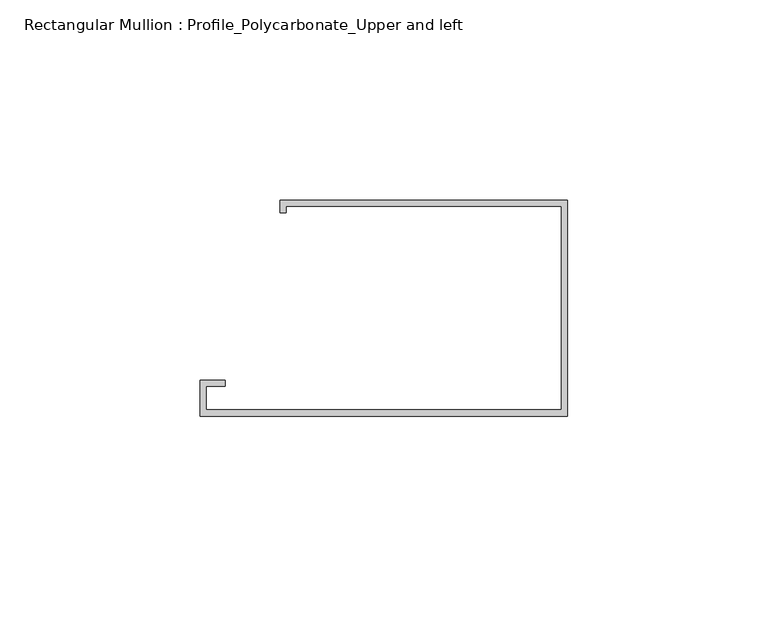
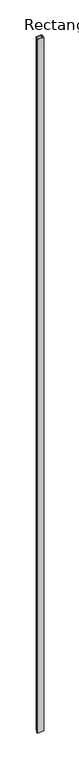
"""IFC4 building model written with IfcOpenShell, lengths in millimetres: member geometry, Rectangular Mullion : Profile_Polycarbonate_Upper and left."""

import ifcopenshell
import ifcopenshell.guid

model = None  # the IFC model being written
_history = None  # IfcOwnerHistory: only IFC2X3 demands one
_inside = {}  # id of a spatial element -> (the spatial element, [elements in it])
_under = {}  # id of a project, library or spatial element -> (it, [spatial elements below it])
_declared = {}  # id of a project -> (the project, [libraries it declares])
_typed = {}  # id of a type object -> (the type object, [elements of that type])
_made_of = {}  # id of a material, layer set ... -> (it, [elements and type objects made of it])


def new_model(schema):
    """Start an empty IFC model of exactly this schema.

    Asked for "IFC4X3", IfcOpenShell would pick the latest addendum, in which some entities
    have other attributes; the version numbers below select the first issue.
    IFC2X3 requires an IfcOwnerHistory on every rooted entity: one is made here for all.
    """
    global model, _history
    if schema == "IFC4X3":
        model = ifcopenshell.file(schema_version=(4, 3, 0, 0))
    else:
        model = ifcopenshell.file(schema=schema)
    _inside.clear()
    _under.clear()
    _declared.clear()
    _typed.clear()
    _made_of.clear()
    _history = None
    if model.schema == "IFC2X3":
        org = make("IfcOrganization", Name="unknown")
        user = make(
            "IfcPersonAndOrganization",
            ThePerson=make("IfcPerson", FamilyName="unknown"),
            TheOrganization=org,
        )
        app = make(
            "IfcApplication",
            ApplicationDeveloper=org,
            Version="unknown",
            ApplicationFullName="unknown",
            ApplicationIdentifier="unknown",
        )
        _history = make(
            "IfcOwnerHistory",
            OwningUser=user,
            OwningApplication=app,
            ChangeAction="ADDED",
            CreationDate=0,
        )
    return model


def make(cls, **values):
    """One entity of the class cls with the attributes given. An attribute that is None is left unset."""
    return model.create_entity(
        cls, **{name: value for name, value in values.items() if value is not None}
    )


def rooted(cls, **values):
    """An entity with a GlobalId (a new one), such as an element, a storey or a relation."""
    return make(cls, GlobalId=ifcopenshell.guid.new(), OwnerHistory=_history, **values)


def si_unit(unit_type, name, prefix=None):
    """IfcSIUnit, for example si_unit("LENGTHUNIT", "METRE", prefix="MILLI")."""
    return make("IfcSIUnit", UnitType=unit_type, Prefix=prefix, Name=name)


def assignment(units):
    """IfcUnitAssignment: the units of a project."""
    return None if units is None else make("IfcUnitAssignment", Units=units)


def point(xyz):
    """IfcCartesianPoint."""
    return None if xyz is None else make("IfcCartesianPoint", Coordinates=xyz)


def direction(xyz):
    """IfcDirection."""
    return None if xyz is None else make("IfcDirection", DirectionRatios=xyz)


def frame(location, z_axis=None, x_axis=None):
    """IfcAxis2Placement3D, a coordinate frame: its origin and axes. An axis left out is left unset."""
    return make(
        "IfcAxis2Placement3D",
        Location=point(location),
        Axis=direction(z_axis),
        RefDirection=direction(x_axis),
    )


def origin():
    """The frame at (0, 0, 0) with its axes left unset."""
    return frame((0.0, 0.0, 0.0))


def place(relative_to, where):
    """IfcLocalPlacement: puts the frame where relative to a parent placement (None: the world)."""
    return make(
        "IfcLocalPlacement", PlacementRelTo=relative_to, RelativePlacement=where
    )


def context(
    kind, dimensions, precision=None, world=None, true_north=None, identifier=None
):
    """IfcGeometricRepresentationContext, for example the 3D "Model" context."""
    return make(
        "IfcGeometricRepresentationContext",
        ContextIdentifier=identifier,
        ContextType=kind,
        CoordinateSpaceDimension=dimensions,
        Precision=precision,
        WorldCoordinateSystem=world,
        TrueNorth=true_north,
    )


def project(units=None, contexts=None):
    """IfcProject with its units and contexts."""
    return rooted(
        "IfcProject",
        Name="project",
        RepresentationContexts=contexts,
        UnitsInContext=assignment(units),
    )


def spatial(cls, under=None, at=None, **own):
    """A site, building, storey or space (cls), placed at a placement, below another one or the project."""
    s = rooted(cls, ObjectPlacement=at, **own)
    if under is not None:
        _under.setdefault(under.id(), (under, []))[1].append(s)
    return s


def polyline(points):
    """IfcPolyline through the points."""
    return make("IfcPolyline", Points=[point(p) for p in points])


def outline(outer, holes=None, kind="AREA"):
    """IfcArbitraryClosedProfileDef: a profile drawn as a closed curve; with holes, ...WithVoids."""
    if holes is None:
        return make("IfcArbitraryClosedProfileDef", ProfileType=kind, OuterCurve=outer)
    return make(
        "IfcArbitraryProfileDefWithVoids",
        ProfileType=kind,
        OuterCurve=outer,
        InnerCurves=holes,
    )


def extrude(swept, where, along, depth):
    """IfcExtrudedAreaSolid: the profile swept, set in the frame where, extruded along a direction by depth."""
    return make(
        "IfcExtrudedAreaSolid",
        SweptArea=swept,
        Position=where,
        ExtrudedDirection=direction(along),
        Depth=depth,
    )


def shape(context_of_items, identifier, shape_type, items):
    """IfcShapeRepresentation: the items that make up one representation, for example the "Body"."""
    return make(
        "IfcShapeRepresentation",
        ContextOfItems=context_of_items,
        RepresentationIdentifier=identifier,
        RepresentationType=shape_type,
        Items=items,
    )


def source(mapping_origin, context_of_items, identifier, shape_type, items):
    """IfcRepresentationMap: a shape defined once, which mapped items show again and again."""
    return make(
        "IfcRepresentationMap",
        MappingOrigin=mapping_origin,
        MappedRepresentation=shape(context_of_items, identifier, shape_type, items),
    )


def transform(
    local_origin,
    x_axis=None,
    y_axis=None,
    z_axis=None,
    scale=None,
    scale2=None,
    scale3=None,
    uniform=True,
):
    """IfcCartesianTransformationOperator3D, or its non-uniform kind. x_axis, y_axis, z_axis: its Axis1, 2, 3."""
    if uniform:
        return make(
            "IfcCartesianTransformationOperator3D",
            Axis1=direction(x_axis),
            Axis2=direction(y_axis),
            LocalOrigin=point(local_origin),
            Scale=scale,
            Axis3=direction(z_axis),
        )
    return make(
        "IfcCartesianTransformationOperator3DnonUniform",
        Axis1=direction(x_axis),
        Axis2=direction(y_axis),
        LocalOrigin=point(local_origin),
        Scale=scale,
        Axis3=direction(z_axis),
        Scale2=scale2,
        Scale3=scale3,
    )


def mapped(mapping_source, mapping_target):
    """IfcMappedItem: shows the shape of a source again, moved by a transform."""
    return make(
        "IfcMappedItem", MappingSource=mapping_source, MappingTarget=mapping_target
    )


def made_of(thing, what):
    """Note that an element or type object is made of a material, layer set ...; save() writes the relation."""
    if what is not None:
        _made_of.setdefault(what.id(), (what, []))[1].append(thing)
    return thing


def element(
    cls,
    number,
    at=None,
    inside=None,
    cuts=None,
    type_object=None,
    material=None,
    context=None,
    identifier="Body",
    shape_type=None,
    held_by="IfcProductDefinitionShape",
    body=None,
    shapes=None,
    **own,
):
    """One element of the class cls, such as IfcWall. Its Tag is "e" and its number.

    at: its placement. inside: the storey or other place that contains it. cuts: it is an
    opening in that element (IfcRelVoidsElement). A single representation is given by context,
    identifier, shape_type and body (its items); several are given by shapes. held_by: the class
    of the entity that holds the representations. save() writes the other relations.
    """
    e = rooted(cls, Tag="e%d" % number, ObjectPlacement=at, **own)
    if body is not None:
        shapes = [shape(context, identifier, shape_type, body)]
    if shapes is not None:
        e.Representation = make(held_by, Representations=shapes)
    if inside is not None:
        _inside.setdefault(inside.id(), (inside, []))[1].append(e)
    if cuts is not None:
        rooted(
            "IfcRelVoidsElement", RelatingBuildingElement=cuts, RelatedOpeningElement=e
        )
    if type_object is not None:
        _typed.setdefault(type_object.id(), (type_object, []))[1].append(e)
    return made_of(e, material)


def aggregate(whole, parts):
    """IfcRelAggregates: a whole, such as a stair, and the parts it consists of."""
    return rooted("IfcRelAggregates", RelatingObject=whole, RelatedObjects=parts)


def save(model, path):
    """Write the relations noted so far, then the file.

    IfcRelAggregates (storeys below a building ...), IfcRelContainedInSpatialStructure (elements
    in a storey), IfcRelDefinesByType, IfcRelAssociatesMaterial and IfcRelDeclares: one each for
    every whole, place, type object, material and project.
    """
    for whole, parts in _under.values():
        aggregate(whole, parts)
    for where, things in _inside.values():
        rooted(
            "IfcRelContainedInSpatialStructure",
            RelatedElements=things,
            RelatingStructure=where,
        )
    for kind, things in _typed.values():
        rooted("IfcRelDefinesByType", RelatedObjects=things, RelatingType=kind)
    for what, things in _made_of.values():
        rooted("IfcRelAssociatesMaterial", RelatedObjects=things, RelatingMaterial=what)
    for by, libraries in _declared.values():
        rooted("IfcRelDeclares", RelatingContext=by, RelatedDefinitions=libraries)
    model.write(path)


def rectangular_mullion_profile_polycarbonate_upper_and_left_15736c9c(model_context):
    return source(origin(), model_context, "Body", "SweptSolid", [
        extrude(outline(polyline([(0.0, -28.984575), (-91.9988, -28.984575), (-91.9988, -19.992975), (-85.6488, -19.992975), (-85.6488, -21.580475), (-90.4113, -21.580475), (-90.4113, -27.397075), (-1.5875, -27.397075), (-1.5875, 23.428325), (-70.3961, 23.428325), (-70.3961, 21.840825), (-71.9836, 21.840825), (-71.9836, 25.015825), (0.0, 25.015825), (0.0, -28.984575)])), frame((0.0, 0.0, -9969.6524), z_axis=(0.0, 0.0, 1.0), x_axis=(1.0, 0.0, 0.0)), (0.0, 0.0, 1.0), 9969.6524),
    ])


if __name__ == "__main__":
    model = new_model("IFC4")
    model_context = context("Model", 3, world=origin())
    ifc_project = project(units=[si_unit("LENGTHUNIT", "METRE", prefix="MILLI")], contexts=[model_context])
    site = spatial("IfcSite", under=ifc_project)
    building = spatial("IfcBuilding", under=site)
    placement = place(None, origin())
    rectangular_mullion_profile_polycarbonate_upper_and_left_shape = rectangular_mullion_profile_polycarbonate_upper_and_left_15736c9c(model_context)
    element("IfcMember", 1, ObjectType="Rectangular Mullion : Profile_Polycarbonate_Upper and left", at=placement, inside=building, context=model_context, shape_type="MappedRepresentation", body=[
        mapped(rectangular_mullion_profile_polycarbonate_upper_and_left_shape, transform((0.0, 0.0, 0.0), x_axis=(1.0, 0.0, 0.0), y_axis=(0.0, 1.0, 0.0), z_axis=(0.0, 0.0, 1.0))),
    ])
    save(model, "model.ifc")

# Revit data of these elements
# Type "Rectangular Mullion : Profile_Polycarbonate_Upper and left"
#   built-in parameter 1007322 = 0.177167 (stored number, unit not read)
#   built-in parameter 1007321 = 0.00520833 (stored number, unit not read)
#   built-in parameter 1007320 = 0 (stored number, unit not read)
